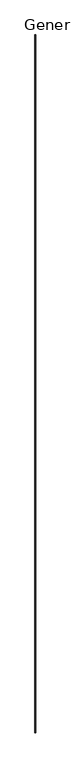
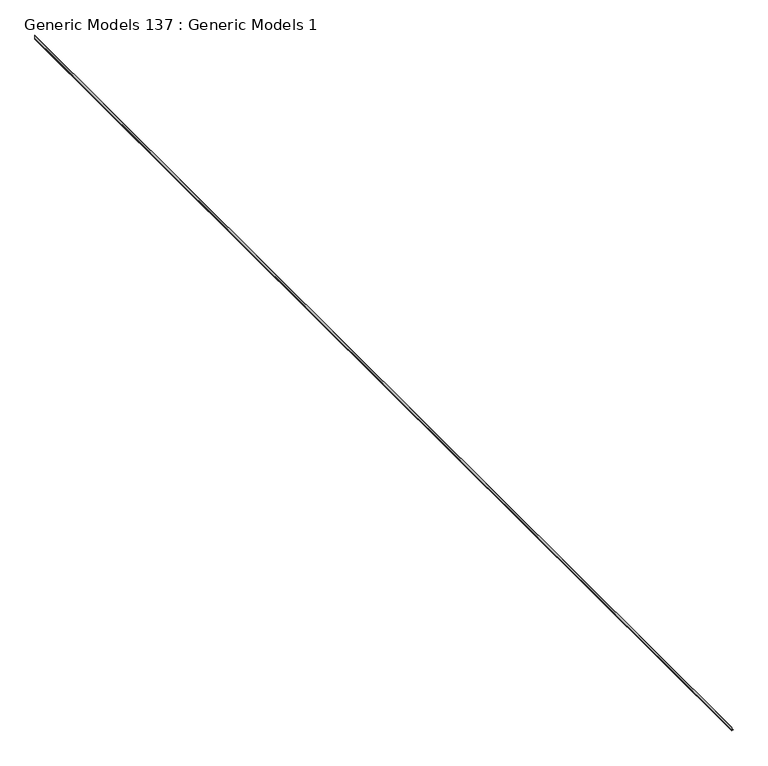
"""IFC4 building model written with IfcOpenShell, lengths in millimetres: proxy geometry, Generic Models 137 : Generic Models 1."""

from ifc_helpers import new_model, si_unit, frame, origin, place, context, project, spatial, polyline, outline, extrude, source, transform, mapped, element, save


def generic_models_137_generic_models_1_b288ad40(model_context):
    return source(origin(), model_context, "Body", "SweptSolid", [
        extrude(outline(polyline([(126958.6728942, 7302.3263705), (126965.4084299, 7281.3713705), (127009.4728942, 7281.3713705), (127009.4728942, 7280.1013705), (126964.4826506, 7280.1013705), (126958.6728942, 7298.1761682), (126953.1727363, 7281.0645656), (126948.0579859, 7280.1013705), (126947.8229543, 7281.349433), (126952.1949461, 7282.1727539), (126958.6728942, 7302.3263705)])), frame((0.0, -7068.1230338, 0.0), z_axis=(0.0, 1.0, 0.0), x_axis=(0.0, 0.0, 1.0)), (0.0, 0.0, 1.0), 19050.0),
    ])


if __name__ == "__main__":
    model = new_model("IFC4")
    model_context = context("Model", 3, world=origin())
    ifc_project = project(units=[si_unit("LENGTHUNIT", "METRE", prefix="MILLI")], contexts=[model_context])
    site = spatial("IfcSite", under=ifc_project)
    building = spatial("IfcBuilding", under=site)
    placement = place(None, origin())
    generic_models_137_generic_models_1_shape = generic_models_137_generic_models_1_b288ad40(model_context)
    element("IfcBuildingElementProxy", 1, Name="Generic Models 137 : Generic Models 1", ObjectType="Generic Models 137 : Generic Models 1", at=placement, inside=building, context=model_context, shape_type="MappedRepresentation", body=[
        mapped(generic_models_137_generic_models_1_shape, transform((0.0, 0.0, 0.0), x_axis=(1.0, 0.0, 0.0), y_axis=(0.0, 1.0, 0.0), z_axis=(0.0, 0.0, 1.0))),
    ])
    save(model, "model.ifc")

# Revit data of these elements
# Element 1 (IfcBuildingElementProxy, "Generic Models 137 : Generic Models 1")
#   Materials on its faces: "_16 GA. COPPER WEEP SCREED W/ MIN. 3 1/2\" ATTACHEMENT FLANGE - LAP UNDERLAYMENT OVER WEED SCREED"
# Materials
#   "_16 GA. COPPER WEEP SCREED W/ MIN. 3 1/2\" ATTACHEMENT FLANGE - LAP UNDERLAYMENT OVER WEED SCREED": class "Generic", colour RGB 253 192 103, transparency 0, Cost = 0
